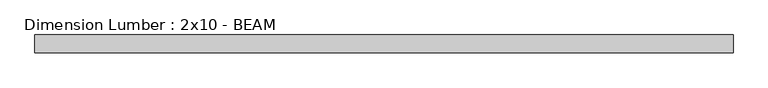
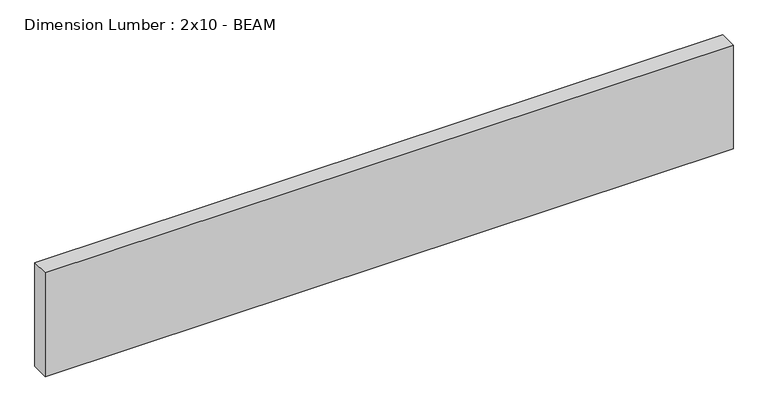
"""IFC4 building model written with IfcOpenShell, lengths in millimetres: beam geometry, Dimension Lumber : 2x10 - BEAM."""

from ifc_helpers import new_model, si_unit, frame, origin, place, context, project, spatial, polyline, outline, extrude, source, transform, mapped, element, save


def dimension_lumber_2x10_beam_e2f510cc(model_context):
    return source(origin(), model_context, "Body", "SweptSolid", [
        extrude(outline(polyline([(736.6, 19.05), (736.6, -19.05), (-736.6, -19.05), (-736.6, 19.05), (736.6, 19.05)])), frame((0.0, 0.0, -117.475), z_axis=(0.0, 0.0, 1.0), x_axis=(1.0, 0.0, 0.0)), (0.0, 0.0, 1.0), 234.95),
    ])


if __name__ == "__main__":
    model = new_model("IFC4")
    model_context = context("Model", 3, world=origin())
    ifc_project = project(units=[si_unit("LENGTHUNIT", "METRE", prefix="MILLI")], contexts=[model_context])
    site = spatial("IfcSite", under=ifc_project)
    building = spatial("IfcBuilding", under=site)
    placement = place(None, origin())
    dimension_lumber_2x10_beam_shape = dimension_lumber_2x10_beam_e2f510cc(model_context)
    element("IfcBeam", 1, ObjectType="Dimension Lumber : 2x10 - BEAM", at=placement, inside=building, context=model_context, shape_type="MappedRepresentation", body=[
        mapped(dimension_lumber_2x10_beam_shape, transform((0.0, 0.0, 0.0), x_axis=(1.0, 0.0, 0.0), y_axis=(0.0, 1.0, 0.0), z_axis=(0.0, 0.0, 1.0))),
    ])
    save(model, "model.ifc")

# Revit data of these elements
# Type "Dimension Lumber : 2x10 - BEAM"
#   Assembly Code = "B10"
#   A = 0.0755556 SF
#   Length [instance default] = 5' - 0"
#   b = 0' - 1 1/2"
#   d = 0' - 9 1/4"
#   Structural Material = (3) SISTERED 2X10s AT BEAM
# Element 1 (IfcBeam, "Dimension Lumber : 2x10 - BEAM")
#   Materials on its faces: "(3) SISTERED 2X10s AT BEAM"
# Materials
#   "(3) SISTERED 2X10s AT BEAM": class "Wood", colour RGB 234 198 147, transparency 0, Description = "Pinus Echinata", Cost = 0
